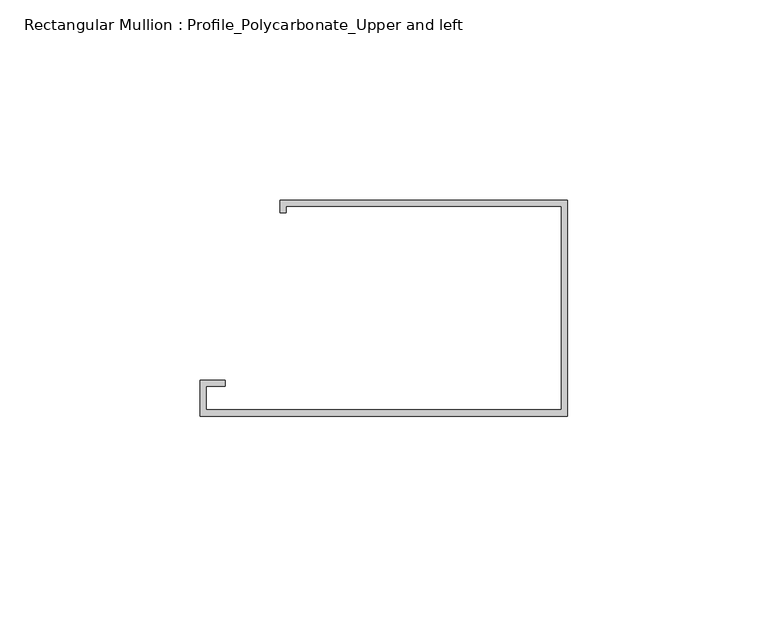
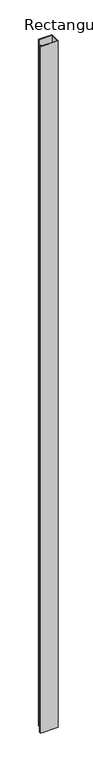
"""IFC4 building model written with IfcOpenShell, lengths in millimetres: member geometry, Rectangular Mullion : Profile_Polycarbonate_Upper and left."""

from ifc_helpers import new_model, si_unit, frame, origin, place, context, project, spatial, polyline, outline, extrude, source, transform, mapped, element, save


def rectangular_mullion_profile_polycarbonate_upper_and_left_6998c9e2(model_context):
    return source(origin(), model_context, "Body", "SweptSolid", [
        extrude(outline(polyline([(0.0, -28.984575), (-91.9988, -28.984575), (-91.9988, -19.992975), (-85.6488, -19.992975), (-85.6488, -21.580475), (-90.4113, -21.580475), (-90.4113, -27.397075), (-1.5875, -27.397075), (-1.5875, 23.428325), (-70.3961, 23.428325), (-70.3961, 21.840825), (-71.9836, 21.840825), (-71.9836, 25.015825), (0.0, 25.015825), (0.0, -28.984575)])), frame((0.0, 0.0, -3804.691455), z_axis=(0.0, 0.0, 1.0), x_axis=(1.0, 0.0, 0.0)), (0.0, 0.0, 1.0), 3804.691455),
    ])


if __name__ == "__main__":
    model = new_model("IFC4")
    model_context = context("Model", 3, world=origin())
    ifc_project = project(units=[si_unit("LENGTHUNIT", "METRE", prefix="MILLI")], contexts=[model_context])
    site = spatial("IfcSite", under=ifc_project)
    building = spatial("IfcBuilding", under=site)
    placement = place(None, origin())
    rectangular_mullion_profile_polycarbonate_upper_and_left_shape = rectangular_mullion_profile_polycarbonate_upper_and_left_6998c9e2(model_context)
    element("IfcMember", 1, ObjectType="Rectangular Mullion : Profile_Polycarbonate_Upper and left", at=placement, inside=building, context=model_context, shape_type="MappedRepresentation", body=[
        mapped(rectangular_mullion_profile_polycarbonate_upper_and_left_shape, transform((0.0, 0.0, 0.0), x_axis=(1.0, 0.0, 0.0), y_axis=(0.0, 1.0, 0.0), z_axis=(0.0, 0.0, 1.0))),
    ])
    save(model, "model.ifc")

# Revit data of these elements
# Type "Rectangular Mullion : Profile_Polycarbonate_Upper and left"
#   built-in parameter 1007322 = 0.177167 (stored number, unit not read)
#   built-in parameter 1007321 = 0.00520833 (stored number, unit not read)
#   built-in parameter 1007320 = 0 (stored number, unit not read)
